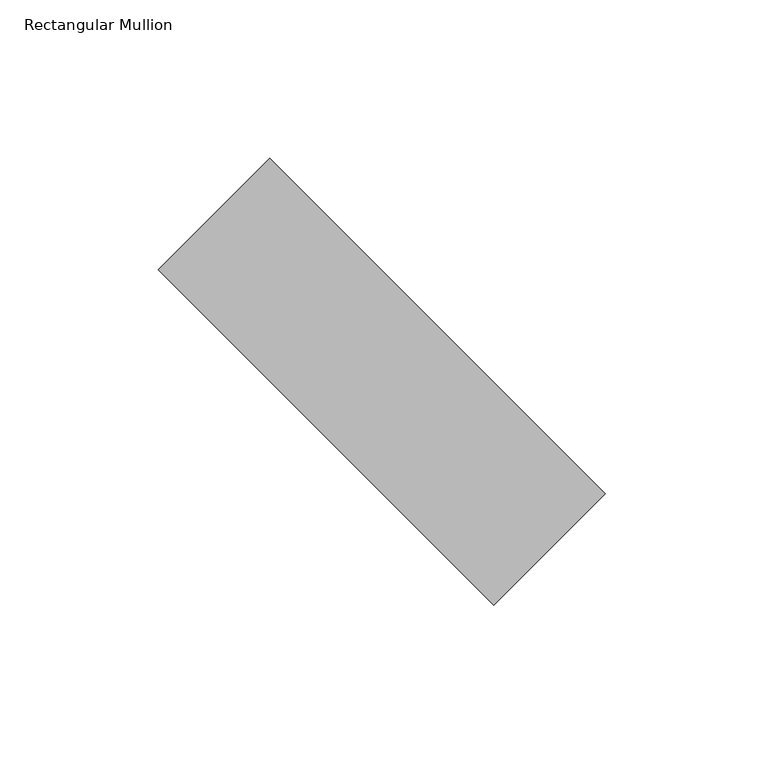
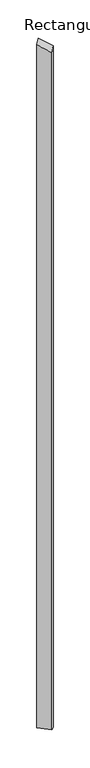
"""IFC4 building model written with IfcOpenShell, lengths in millimetres: member geometry, Rectangular Mullion : tilted mullions."""

import ifcopenshell
import ifcopenshell.guid

model = None  # the IFC model being written
_history = None  # IfcOwnerHistory: only IFC2X3 demands one
_inside = {}  # id of a spatial element -> (the spatial element, [elements in it])
_under = {}  # id of a project, library or spatial element -> (it, [spatial elements below it])
_declared = {}  # id of a project -> (the project, [libraries it declares])
_typed = {}  # id of a type object -> (the type object, [elements of that type])
_made_of = {}  # id of a material, layer set ... -> (it, [elements and type objects made of it])


def new_model(schema):
    """Start an empty IFC model of exactly this schema.

    Asked for "IFC4X3", IfcOpenShell would pick the latest addendum, in which some entities
    have other attributes; the version numbers below select the first issue.
    IFC2X3 requires an IfcOwnerHistory on every rooted entity: one is made here for all.
    """
    global model, _history
    if schema == "IFC4X3":
        model = ifcopenshell.file(schema_version=(4, 3, 0, 0))
    else:
        model = ifcopenshell.file(schema=schema)
    _inside.clear()
    _under.clear()
    _declared.clear()
    _typed.clear()
    _made_of.clear()
    _history = None
    if model.schema == "IFC2X3":
        org = make("IfcOrganization", Name="unknown")
        user = make(
            "IfcPersonAndOrganization",
            ThePerson=make("IfcPerson", FamilyName="unknown"),
            TheOrganization=org,
        )
        app = make(
            "IfcApplication",
            ApplicationDeveloper=org,
            Version="unknown",
            ApplicationFullName="unknown",
            ApplicationIdentifier="unknown",
        )
        _history = make(
            "IfcOwnerHistory",
            OwningUser=user,
            OwningApplication=app,
            ChangeAction="ADDED",
            CreationDate=0,
        )
    return model


def make(cls, **values):
    """One entity of the class cls with the attributes given. An attribute that is None is left unset."""
    return model.create_entity(
        cls, **{name: value for name, value in values.items() if value is not None}
    )


def rooted(cls, **values):
    """An entity with a GlobalId (a new one), such as an element, a storey or a relation."""
    return make(cls, GlobalId=ifcopenshell.guid.new(), OwnerHistory=_history, **values)


def si_unit(unit_type, name, prefix=None):
    """IfcSIUnit, for example si_unit("LENGTHUNIT", "METRE", prefix="MILLI")."""
    return make("IfcSIUnit", UnitType=unit_type, Prefix=prefix, Name=name)


def assignment(units):
    """IfcUnitAssignment: the units of a project."""
    return None if units is None else make("IfcUnitAssignment", Units=units)


def point(xyz):
    """IfcCartesianPoint."""
    return None if xyz is None else make("IfcCartesianPoint", Coordinates=xyz)


def direction(xyz):
    """IfcDirection."""
    return None if xyz is None else make("IfcDirection", DirectionRatios=xyz)


def frame(location, z_axis=None, x_axis=None):
    """IfcAxis2Placement3D, a coordinate frame: its origin and axes. An axis left out is left unset."""
    return make(
        "IfcAxis2Placement3D",
        Location=point(location),
        Axis=direction(z_axis),
        RefDirection=direction(x_axis),
    )


def origin():
    """The frame at (0, 0, 0) with its axes left unset."""
    return frame((0.0, 0.0, 0.0))


def place(relative_to, where):
    """IfcLocalPlacement: puts the frame where relative to a parent placement (None: the world)."""
    return make(
        "IfcLocalPlacement", PlacementRelTo=relative_to, RelativePlacement=where
    )


def context(
    kind, dimensions, precision=None, world=None, true_north=None, identifier=None
):
    """IfcGeometricRepresentationContext, for example the 3D "Model" context."""
    return make(
        "IfcGeometricRepresentationContext",
        ContextIdentifier=identifier,
        ContextType=kind,
        CoordinateSpaceDimension=dimensions,
        Precision=precision,
        WorldCoordinateSystem=world,
        TrueNorth=true_north,
    )


def project(units=None, contexts=None):
    """IfcProject with its units and contexts."""
    return rooted(
        "IfcProject",
        Name="project",
        RepresentationContexts=contexts,
        UnitsInContext=assignment(units),
    )


def spatial(cls, under=None, at=None, **own):
    """A site, building, storey or space (cls), placed at a placement, below another one or the project."""
    s = rooted(cls, ObjectPlacement=at, **own)
    if under is not None:
        _under.setdefault(under.id(), (under, []))[1].append(s)
    return s


def faces_of(points, faces, orient=None, outer=None):
    """IfcFace entities. A face is a list of loops; a loop is a list of indices into points, from 0.

    orient and outer hold one flag for each loop. By default every Orientation is true, the
    first loop of a face is its IfcFaceOuterBound and the others are IfcFaceBound.
    """
    made = []
    for i, loops in enumerate(faces):
        bounds = []
        for j, loop in enumerate(loops):
            is_outer = j == 0 if outer is None else outer[i][j]
            bounds.append(
                make(
                    "IfcFaceOuterBound" if is_outer else "IfcFaceBound",
                    Bound=make("IfcPolyLoop", Polygon=[points[k] for k in loop]),
                    Orientation=True if orient is None else orient[i][j],
                )
            )
        made.append(make("IfcFace", Bounds=bounds))
    return made


def faceted_brep(points, faces, orient=None, outer=None, voids=None):
    """IfcFacetedBrep: a solid bounded by flat faces; with voids (closed shells), ...WithVoids."""
    shared = [point(p) for p in points]
    hull = make("IfcClosedShell", CfsFaces=faces_of(shared, faces, orient, outer))
    if voids is None:
        return make("IfcFacetedBrep", Outer=hull)
    return make(
        "IfcFacetedBrepWithVoids",
        Outer=hull,
        Voids=[
            make(cls, CfsFaces=faces_of(shared, fs, o, b)) for cls, fs, o, b in voids
        ],
    )


def shape(context_of_items, identifier, shape_type, items):
    """IfcShapeRepresentation: the items that make up one representation, for example the "Body"."""
    return make(
        "IfcShapeRepresentation",
        ContextOfItems=context_of_items,
        RepresentationIdentifier=identifier,
        RepresentationType=shape_type,
        Items=items,
    )


def source(mapping_origin, context_of_items, identifier, shape_type, items):
    """IfcRepresentationMap: a shape defined once, which mapped items show again and again."""
    return make(
        "IfcRepresentationMap",
        MappingOrigin=mapping_origin,
        MappedRepresentation=shape(context_of_items, identifier, shape_type, items),
    )


def transform(
    local_origin,
    x_axis=None,
    y_axis=None,
    z_axis=None,
    scale=None,
    scale2=None,
    scale3=None,
    uniform=True,
):
    """IfcCartesianTransformationOperator3D, or its non-uniform kind. x_axis, y_axis, z_axis: its Axis1, 2, 3."""
    if uniform:
        return make(
            "IfcCartesianTransformationOperator3D",
            Axis1=direction(x_axis),
            Axis2=direction(y_axis),
            LocalOrigin=point(local_origin),
            Scale=scale,
            Axis3=direction(z_axis),
        )
    return make(
        "IfcCartesianTransformationOperator3DnonUniform",
        Axis1=direction(x_axis),
        Axis2=direction(y_axis),
        LocalOrigin=point(local_origin),
        Scale=scale,
        Axis3=direction(z_axis),
        Scale2=scale2,
        Scale3=scale3,
    )


def mapped(mapping_source, mapping_target):
    """IfcMappedItem: shows the shape of a source again, moved by a transform."""
    return make(
        "IfcMappedItem", MappingSource=mapping_source, MappingTarget=mapping_target
    )


def made_of(thing, what):
    """Note that an element or type object is made of a material, layer set ...; save() writes the relation."""
    if what is not None:
        _made_of.setdefault(what.id(), (what, []))[1].append(thing)
    return thing


def element(
    cls,
    number,
    at=None,
    inside=None,
    cuts=None,
    type_object=None,
    material=None,
    context=None,
    identifier="Body",
    shape_type=None,
    held_by="IfcProductDefinitionShape",
    body=None,
    shapes=None,
    **own,
):
    """One element of the class cls, such as IfcWall. Its Tag is "e" and its number.

    at: its placement. inside: the storey or other place that contains it. cuts: it is an
    opening in that element (IfcRelVoidsElement). A single representation is given by context,
    identifier, shape_type and body (its items); several are given by shapes. held_by: the class
    of the entity that holds the representations. save() writes the other relations.
    """
    e = rooted(cls, Tag="e%d" % number, ObjectPlacement=at, **own)
    if body is not None:
        shapes = [shape(context, identifier, shape_type, body)]
    if shapes is not None:
        e.Representation = make(held_by, Representations=shapes)
    if inside is not None:
        _inside.setdefault(inside.id(), (inside, []))[1].append(e)
    if cuts is not None:
        rooted(
            "IfcRelVoidsElement", RelatingBuildingElement=cuts, RelatedOpeningElement=e
        )
    if type_object is not None:
        _typed.setdefault(type_object.id(), (type_object, []))[1].append(e)
    return made_of(e, material)


def aggregate(whole, parts):
    """IfcRelAggregates: a whole, such as a stair, and the parts it consists of."""
    return rooted("IfcRelAggregates", RelatingObject=whole, RelatedObjects=parts)


def save(model, path):
    """Write the relations noted so far, then the file.

    IfcRelAggregates (storeys below a building ...), IfcRelContainedInSpatialStructure (elements
    in a storey), IfcRelDefinesByType, IfcRelAssociatesMaterial and IfcRelDeclares: one each for
    every whole, place, type object, material and project.
    """
    for whole, parts in _under.values():
        aggregate(whole, parts)
    for where, things in _inside.values():
        rooted(
            "IfcRelContainedInSpatialStructure",
            RelatedElements=things,
            RelatingStructure=where,
        )
    for kind, things in _typed.values():
        rooted("IfcRelDefinesByType", RelatedObjects=things, RelatingType=kind)
    for what, things in _made_of.values():
        rooted("IfcRelAssociatesMaterial", RelatedObjects=things, RelatingMaterial=what)
    for by, libraries in _declared.values():
        rooted("IfcRelDeclares", RelatingContext=by, RelatedDefinitions=libraries)
    model.write(path)


def rectangular_mullion_345c46c6(model_context):
    return source(origin(), model_context, "Body", "Brep", [
        faceted_brep([(-35.3553391, 70.7106781, -7999.7689278), (70.7106781, -35.3553391, -7999.7689278), (35.3553391, -70.7106781, -7999.7689278), (-70.7106781, 35.3553391, -7999.7689278), (-70.7106781, 35.3553391, 10.2368528), (-35.3553391, 70.7106781, 55.2243041), (35.3553391, -70.7106781, -55.2243041), (70.7106781, -35.3553391, -10.2368528)], [[[0, 1, 2, 3]], [[4, 5, 0, 3]], [[6, 4, 3, 2]], [[7, 6, 2, 1]], [[5, 7, 1, 0]], [[5, 4, 6, 7]]]),
    ])


if __name__ == "__main__":
    model = new_model("IFC4")
    model_context = context("Model", 3, world=origin())
    ifc_project = project(units=[si_unit("LENGTHUNIT", "METRE", prefix="MILLI")], contexts=[model_context])
    site = spatial("IfcSite", under=ifc_project)
    building = spatial("IfcBuilding", under=site)
    placement = place(None, origin())
    rectangular_mullion_shape = rectangular_mullion_345c46c6(model_context)
    element("IfcMember", 1, ObjectType="Rectangular Mullion : tilted mullions", at=placement, inside=building, context=model_context, shape_type="MappedRepresentation", body=[
        mapped(rectangular_mullion_shape, transform((0.0, 0.0, 0.0), x_axis=(1.0, 0.0, 0.0), y_axis=(0.0, 1.0, 0.0), z_axis=(0.0, 0.0, 1.0))),
    ])
    save(model, "model.ifc")

# Revit data of these elements
# Type "Rectangular Mullion : tilted mullions"
#   built-in parameter 1007304 = 0.492126 (stored number, unit not read)
#   built-in parameter 1007301 = 0.082021 (stored number, unit not read)
#   built-in parameter 1007300 = 0.082021 (stored number, unit not read)
# Element 1 (IfcMember, "Rectangular Mullion : tilted mullions")
#   Materials on its faces: "Aluminum"
# Materials
#   "Aluminum": class "Metal", colour RGB 244 244 244, transparency 0, Description = "Aluminum 6061", Cost = 0
